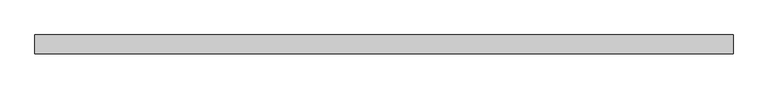
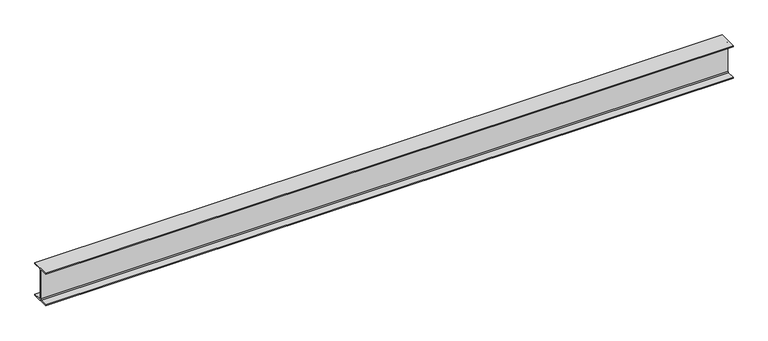
"""IFC4 building model written with IfcOpenShell, lengths in millimetres: beam geometry, Old_Steel Beam_H-KSD3502 : H_SB_ASB_H-400×200x8x13."""

from ifc_helpers import new_model, si_unit, point, frame, frame_2d, origin, place, context, project, spatial, polyline, circle_curve, trimmed, segment, composite_curve, outline, extrude, source, transform, mapped, element, save


def beam_a3ba6330(model_context):
    return source(origin(), model_context, "Body", "SweptSolid", [
        extrude(outline(composite_curve([segment(polyline([(82.5, -141.5), (82.5, -151.7), (-82.5, -151.7), (-82.5, -141.5), (-11.9, -141.5)]), True, "CONTINUOUS"), segment(trimmed(circle_curve(frame_2d((-11.9, -132.6)), 8.9), [point((-11.9, -141.5))], [point((-3.0, -132.6))], True, "CARTESIAN"), True, "CONTINUOUS"), segment(polyline([(-3.0, -132.6), (-3.0, 132.6)]), True, "CONTINUOUS"), segment(trimmed(circle_curve(frame_2d((-11.9, 132.6)), 8.9), [point((-3.0, 132.6))], [point((-11.9, 141.5))], True, "CARTESIAN"), True, "CONTINUOUS"), segment(polyline([(-11.9, 141.5), (-82.5, 141.5), (-82.5, 151.7), (82.5, 151.7), (82.5, 141.5), (11.9, 141.5)]), True, "CONTINUOUS"), segment(trimmed(circle_curve(frame_2d((11.9, 132.6)), 8.9), [point((11.9, 141.5))], [point((3.0, 132.6))], True, "CARTESIAN"), True, "CONTINUOUS"), segment(polyline([(3.0, 132.6), (3.0, -132.6)]), True, "CONTINUOUS"), segment(trimmed(circle_curve(frame_2d((11.9, -132.6)), 8.9), [point((3.0, -132.6))], [point((11.9, -141.5))], True, "CARTESIAN"), True, "CONTINUOUS"), segment(polyline([(11.9, -141.5), (82.5, -141.5)]), True, "CONTINUOUS")], self_intersect=False)), frame((-3007.3488581, 0.0, 0.0), z_axis=(1.0, 0.0, 0.0), x_axis=(0.0, 1.0, 0.0)), (0.0, 0.0, 1.0), 6044.6488581),
    ])


if __name__ == "__main__":
    model = new_model("IFC4")
    model_context = context("Model", 3, world=origin())
    ifc_project = project(units=[si_unit("LENGTHUNIT", "METRE", prefix="MILLI")], contexts=[model_context])
    site = spatial("IfcSite", under=ifc_project)
    building = spatial("IfcBuilding", under=site)
    placement = place(None, origin())
    beam_shape = beam_a3ba6330(model_context)
    element("IfcBeam", 1, ObjectType="Old_Steel Beam_H-KSD3502 : H_SB_ASB_H-400×200x8x13", at=placement, inside=building, context=model_context, shape_type="MappedRepresentation", body=[
        mapped(beam_shape, transform((0.0, 0.0, 0.0), x_axis=(1.0, 0.0, 0.0), y_axis=(0.0, 1.0, 0.0), z_axis=(0.0, 0.0, 1.0))),
    ])
    save(model, "model.ifc")

# Revit data of these elements
# Type "Old_Steel Beam_H-KSD3502 : H_SB_ASB_H-400×200x8x13"
#   Width = 20.0 cm
#   Web Thickness = 0.8 cm
#   Web Fillet = 1.6 cm
#   Warping Constant = 648999.0 cm⁶
#   Torsional Moment of Inertia = 35.8981 cm⁴
#   Torsional Modulus = 1.0 cm³
#   Section Area = 84.12 cm²
#   Plastic Modulus weak axis = 268.0 cm³
#   Plastic Modulus strong axis = 1330.0 cm³
#   Perimeter = 1.56 m²/m
#   Nominal Weight = 66.00 kgf/m
#   Moment of Inertia weak axis = 1740.00 cm⁴
#   Moment of Inertia strong axis = 23700.00 cm⁴
#   Height = 40.0 cm
#   Flange Thickness = 1.3 cm
#   Elastic Modulus weak axis = 174.0 cm³
#   Elastic Modulus strong axis = 1190.0 cm³
#   Centroid Vertical = 20.0 cm
#   Centroid Horizontal = 10.0 cm
#   Length [instance default] = 1.5240 m
#   Structural Material [instance default] = Steel, 45-345
#   Assembly Code = ""
# Element 1 (IfcBeam, "Old_Steel Beam_H-KSD3502 : H_SB_ASB_H-400×200x8x13")
#   Structural Material = none
# Materials
#   "Steel, 45-345": class "Metal", colour RGB 189 187 185, transparency 0, Description = "Steel 345 MPa", Cost = 0
